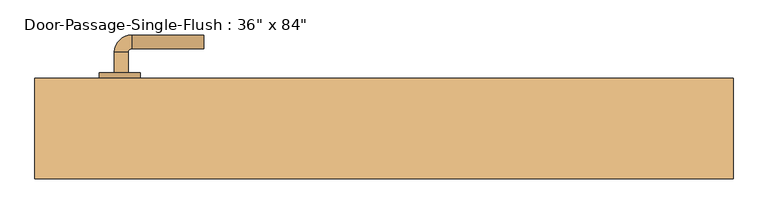
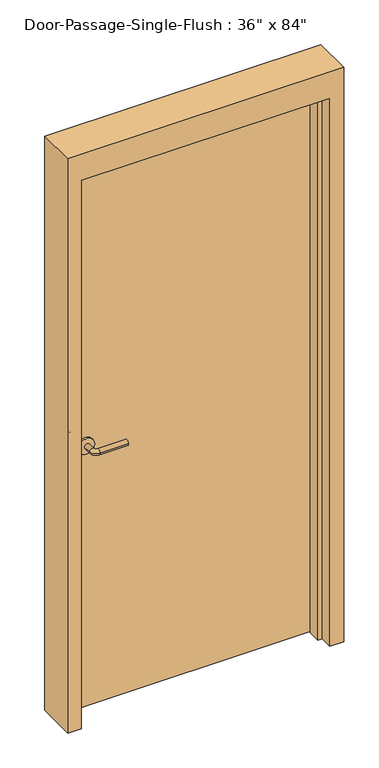
"""IFC4 building model written with IfcOpenShell, lengths in millimetres: door geometry."""

import ifcopenshell
import ifcopenshell.guid

model = None  # the IFC model being written
_history = None  # IfcOwnerHistory: only IFC2X3 demands one
_inside = {}  # id of a spatial element -> (the spatial element, [elements in it])
_under = {}  # id of a project, library or spatial element -> (it, [spatial elements below it])
_declared = {}  # id of a project -> (the project, [libraries it declares])
_typed = {}  # id of a type object -> (the type object, [elements of that type])
_made_of = {}  # id of a material, layer set ... -> (it, [elements and type objects made of it])


def new_model(schema):
    """Start an empty IFC model of exactly this schema.

    Asked for "IFC4X3", IfcOpenShell would pick the latest addendum, in which some entities
    have other attributes; the version numbers below select the first issue.
    IFC2X3 requires an IfcOwnerHistory on every rooted entity: one is made here for all.
    """
    global model, _history
    if schema == "IFC4X3":
        model = ifcopenshell.file(schema_version=(4, 3, 0, 0))
    else:
        model = ifcopenshell.file(schema=schema)
    _inside.clear()
    _under.clear()
    _declared.clear()
    _typed.clear()
    _made_of.clear()
    _history = None
    if model.schema == "IFC2X3":
        org = make("IfcOrganization", Name="unknown")
        user = make(
            "IfcPersonAndOrganization",
            ThePerson=make("IfcPerson", FamilyName="unknown"),
            TheOrganization=org,
        )
        app = make(
            "IfcApplication",
            ApplicationDeveloper=org,
            Version="unknown",
            ApplicationFullName="unknown",
            ApplicationIdentifier="unknown",
        )
        _history = make(
            "IfcOwnerHistory",
            OwningUser=user,
            OwningApplication=app,
            ChangeAction="ADDED",
            CreationDate=0,
        )
    return model


def make(cls, **values):
    """One entity of the class cls with the attributes given. An attribute that is None is left unset."""
    return model.create_entity(
        cls, **{name: value for name, value in values.items() if value is not None}
    )


def rooted(cls, **values):
    """An entity with a GlobalId (a new one), such as an element, a storey or a relation."""
    return make(cls, GlobalId=ifcopenshell.guid.new(), OwnerHistory=_history, **values)


def si_unit(unit_type, name, prefix=None):
    """IfcSIUnit, for example si_unit("LENGTHUNIT", "METRE", prefix="MILLI")."""
    return make("IfcSIUnit", UnitType=unit_type, Prefix=prefix, Name=name)


def assignment(units):
    """IfcUnitAssignment: the units of a project."""
    return None if units is None else make("IfcUnitAssignment", Units=units)


def point(xyz):
    """IfcCartesianPoint."""
    return None if xyz is None else make("IfcCartesianPoint", Coordinates=xyz)


def direction(xyz):
    """IfcDirection."""
    return None if xyz is None else make("IfcDirection", DirectionRatios=xyz)


def frame(location, z_axis=None, x_axis=None):
    """IfcAxis2Placement3D, a coordinate frame: its origin and axes. An axis left out is left unset."""
    return make(
        "IfcAxis2Placement3D",
        Location=point(location),
        Axis=direction(z_axis),
        RefDirection=direction(x_axis),
    )


def frame_2d(location, x_axis=None):
    """IfcAxis2Placement2D, a coordinate frame in the plane: its origin and x axis."""
    return make(
        "IfcAxis2Placement2D", Location=point(location), RefDirection=direction(x_axis)
    )


def origin():
    """The frame at (0, 0, 0) with its axes left unset."""
    return frame((0.0, 0.0, 0.0))


def origin_with_axes():
    """The frame at (0, 0, 0) with the z axis (0, 0, 1) and the x axis (1, 0, 0) written out."""
    return frame((0.0, 0.0, 0.0), z_axis=(0.0, 0.0, 1.0), x_axis=(1.0, 0.0, 0.0))


def place(relative_to, where):
    """IfcLocalPlacement: puts the frame where relative to a parent placement (None: the world)."""
    return make(
        "IfcLocalPlacement", PlacementRelTo=relative_to, RelativePlacement=where
    )


def context(
    kind, dimensions, precision=None, world=None, true_north=None, identifier=None
):
    """IfcGeometricRepresentationContext, for example the 3D "Model" context."""
    return make(
        "IfcGeometricRepresentationContext",
        ContextIdentifier=identifier,
        ContextType=kind,
        CoordinateSpaceDimension=dimensions,
        Precision=precision,
        WorldCoordinateSystem=world,
        TrueNorth=true_north,
    )


def project(units=None, contexts=None):
    """IfcProject with its units and contexts."""
    return rooted(
        "IfcProject",
        Name="project",
        RepresentationContexts=contexts,
        UnitsInContext=assignment(units),
    )


def spatial(cls, under=None, at=None, **own):
    """A site, building, storey or space (cls), placed at a placement, below another one or the project."""
    s = rooted(cls, ObjectPlacement=at, **own)
    if under is not None:
        _under.setdefault(under.id(), (under, []))[1].append(s)
    return s


def polyline(points):
    """IfcPolyline through the points."""
    return make("IfcPolyline", Points=[point(p) for p in points])


def circle_curve(where, radius):
    """IfcCircle in the frame where."""
    return make("IfcCircle", Position=where, Radius=radius)


def ellipse_curve(where, semi_axis1, semi_axis2):
    """IfcEllipse in the frame where."""
    return make(
        "IfcEllipse", Position=where, SemiAxis1=semi_axis1, SemiAxis2=semi_axis2
    )


def trimmed(basis, trim1, trim2, sense, master):
    """IfcTrimmedCurve: the piece of a basis curve between two trims."""
    return make(
        "IfcTrimmedCurve",
        BasisCurve=basis,
        Trim1=trim1,
        Trim2=trim2,
        SenseAgreement=sense,
        MasterRepresentation=master,
    )


def segment(curve, same_sense, transition):
    """IfcCompositeCurveSegment."""
    return make(
        "IfcCompositeCurveSegment",
        Transition=transition,
        SameSense=same_sense,
        ParentCurve=curve,
    )


def composite_curve(segments, self_intersect=None):
    """IfcCompositeCurve: segments joined end to end."""
    return make("IfcCompositeCurve", Segments=segments, SelfIntersect=self_intersect)


def outline(outer, holes=None, kind="AREA"):
    """IfcArbitraryClosedProfileDef: a profile drawn as a closed curve; with holes, ...WithVoids."""
    if holes is None:
        return make("IfcArbitraryClosedProfileDef", ProfileType=kind, OuterCurve=outer)
    return make(
        "IfcArbitraryProfileDefWithVoids",
        ProfileType=kind,
        OuterCurve=outer,
        InnerCurves=holes,
    )


def extrude(swept, where, along, depth):
    """IfcExtrudedAreaSolid: the profile swept, set in the frame where, extruded along a direction by depth."""
    return make(
        "IfcExtrudedAreaSolid",
        SweptArea=swept,
        Position=where,
        ExtrudedDirection=direction(along),
        Depth=depth,
    )


def faces_of(points, faces, orient=None, outer=None):
    """IfcFace entities. A face is a list of loops; a loop is a list of indices into points, from 0.

    orient and outer hold one flag for each loop. By default every Orientation is true, the
    first loop of a face is its IfcFaceOuterBound and the others are IfcFaceBound.
    """
    made = []
    for i, loops in enumerate(faces):
        bounds = []
        for j, loop in enumerate(loops):
            is_outer = j == 0 if outer is None else outer[i][j]
            bounds.append(
                make(
                    "IfcFaceOuterBound" if is_outer else "IfcFaceBound",
                    Bound=make("IfcPolyLoop", Polygon=[points[k] for k in loop]),
                    Orientation=True if orient is None else orient[i][j],
                )
            )
        made.append(make("IfcFace", Bounds=bounds))
    return made


def faceted_brep(points, faces, orient=None, outer=None, voids=None):
    """IfcFacetedBrep: a solid bounded by flat faces; with voids (closed shells), ...WithVoids."""
    shared = [point(p) for p in points]
    hull = make("IfcClosedShell", CfsFaces=faces_of(shared, faces, orient, outer))
    if voids is None:
        return make("IfcFacetedBrep", Outer=hull)
    return make(
        "IfcFacetedBrepWithVoids",
        Outer=hull,
        Voids=[
            make(cls, CfsFaces=faces_of(shared, fs, o, b)) for cls, fs, o, b in voids
        ],
    )


def shape(context_of_items, identifier, shape_type, items):
    """IfcShapeRepresentation: the items that make up one representation, for example the "Body"."""
    return make(
        "IfcShapeRepresentation",
        ContextOfItems=context_of_items,
        RepresentationIdentifier=identifier,
        RepresentationType=shape_type,
        Items=items,
    )


def source(mapping_origin, context_of_items, identifier, shape_type, items):
    """IfcRepresentationMap: a shape defined once, which mapped items show again and again."""
    return make(
        "IfcRepresentationMap",
        MappingOrigin=mapping_origin,
        MappedRepresentation=shape(context_of_items, identifier, shape_type, items),
    )


def transform(
    local_origin,
    x_axis=None,
    y_axis=None,
    z_axis=None,
    scale=None,
    scale2=None,
    scale3=None,
    uniform=True,
):
    """IfcCartesianTransformationOperator3D, or its non-uniform kind. x_axis, y_axis, z_axis: its Axis1, 2, 3."""
    if uniform:
        return make(
            "IfcCartesianTransformationOperator3D",
            Axis1=direction(x_axis),
            Axis2=direction(y_axis),
            LocalOrigin=point(local_origin),
            Scale=scale,
            Axis3=direction(z_axis),
        )
    return make(
        "IfcCartesianTransformationOperator3DnonUniform",
        Axis1=direction(x_axis),
        Axis2=direction(y_axis),
        LocalOrigin=point(local_origin),
        Scale=scale,
        Axis3=direction(z_axis),
        Scale2=scale2,
        Scale3=scale3,
    )


def mapped(mapping_source, mapping_target):
    """IfcMappedItem: shows the shape of a source again, moved by a transform."""
    return make(
        "IfcMappedItem", MappingSource=mapping_source, MappingTarget=mapping_target
    )


def made_of(thing, what):
    """Note that an element or type object is made of a material, layer set ...; save() writes the relation."""
    if what is not None:
        _made_of.setdefault(what.id(), (what, []))[1].append(thing)
    return thing


def element(
    cls,
    number,
    at=None,
    inside=None,
    cuts=None,
    type_object=None,
    material=None,
    context=None,
    identifier="Body",
    shape_type=None,
    held_by="IfcProductDefinitionShape",
    body=None,
    shapes=None,
    **own,
):
    """One element of the class cls, such as IfcWall. Its Tag is "e" and its number.

    at: its placement. inside: the storey or other place that contains it. cuts: it is an
    opening in that element (IfcRelVoidsElement). A single representation is given by context,
    identifier, shape_type and body (its items); several are given by shapes. held_by: the class
    of the entity that holds the representations. save() writes the other relations.
    """
    e = rooted(cls, Tag="e%d" % number, ObjectPlacement=at, **own)
    if body is not None:
        shapes = [shape(context, identifier, shape_type, body)]
    if shapes is not None:
        e.Representation = make(held_by, Representations=shapes)
    if inside is not None:
        _inside.setdefault(inside.id(), (inside, []))[1].append(e)
    if cuts is not None:
        rooted(
            "IfcRelVoidsElement", RelatingBuildingElement=cuts, RelatedOpeningElement=e
        )
    if type_object is not None:
        _typed.setdefault(type_object.id(), (type_object, []))[1].append(e)
    return made_of(e, material)


def aggregate(whole, parts):
    """IfcRelAggregates: a whole, such as a stair, and the parts it consists of."""
    return rooted("IfcRelAggregates", RelatingObject=whole, RelatedObjects=parts)


def save(model, path):
    """Write the relations noted so far, then the file.

    IfcRelAggregates (storeys below a building ...), IfcRelContainedInSpatialStructure (elements
    in a storey), IfcRelDefinesByType, IfcRelAssociatesMaterial and IfcRelDeclares: one each for
    every whole, place, type object, material and project.
    """
    for whole, parts in _under.values():
        aggregate(whole, parts)
    for where, things in _inside.values():
        rooted(
            "IfcRelContainedInSpatialStructure",
            RelatedElements=things,
            RelatingStructure=where,
        )
    for kind, things in _typed.values():
        rooted("IfcRelDefinesByType", RelatedObjects=things, RelatingType=kind)
    for what, things in _made_of.values():
        rooted("IfcRelAssociatesMaterial", RelatedObjects=things, RelatingMaterial=what)
    for by, libraries in _declared.values():
        rooted("IfcRelDeclares", RelatingContext=by, RelatedDefinitions=libraries)
    model.write(path)


def plane_surface(at):
    """IfcPlane: the flat surface through the origin of the frame at, square to its z axis."""
    return make("IfcPlane", Position=at)


def cylinder_surface(at, radius):
    """IfcCylindricalSurface: all points at the distance radius from the z axis of the frame at."""
    return make("IfcCylindricalSurface", Position=at, Radius=radius)


def revolved_surface(curve, axis_point, axis_direction):
    """IfcSurfaceOfRevolution: the curve turned about the line through axis_point along axis_direction."""
    return make(
        "IfcSurfaceOfRevolution",
        SweptCurve=make("IfcArbitraryOpenProfileDef", ProfileType="CURVE", Curve=curve),
        AxisPosition=make("IfcAxis1Placement", Location=point(axis_point), Axis=direction(axis_direction)),
    )


def advanced_brep(points, edges, surfaces, faces):
    """IfcAdvancedBrep: a solid bounded by faces that lie on surfaces and meet in shared edges.

    An edge is (start, end): straight between two places in points (the first is 0);
    or (start, end, curve); or (start, end, curve, False) where it runs against its curve.
    A face is (place in surfaces, loops), or (place, loops, False) where it looks against
    its surface's normal. A loop lists edges by number (the first is 1), with a minus sign
    where the edge is run from its end to its start. The first loop is the outer one.
    """
    corners = [point(p) for p in points]
    vertices = [make("IfcVertexPoint", VertexGeometry=c) for c in corners]
    made = []
    for start, end, *more in edges:
        made.append(
            make(
                "IfcEdgeCurve",
                EdgeStart=vertices[start],
                EdgeEnd=vertices[end],
                EdgeGeometry=more[0] if more else make("IfcPolyline", Points=[corners[start], corners[end]]),
                SameSense=more[1] if len(more) > 1 else True,
            )
        )
    hull = []
    for where, loops, *sense in faces:
        bounds = []
        for j, loop in enumerate(loops):
            ring = [make("IfcOrientedEdge", EdgeElement=made[abs(k) - 1], Orientation=k > 0) for k in loop]
            bounds.append(
                make(
                    "IfcFaceOuterBound" if j == 0 else "IfcFaceBound",
                    Bound=make("IfcEdgeLoop", EdgeList=ring),
                    Orientation=True,
                )
            )
        hull.append(make("IfcAdvancedFace", Bounds=bounds, FaceSurface=surfaces[where], SameSense=sense[0] if sense else True))
    return make("IfcAdvancedBrep", Outer=make("IfcClosedShell", CfsFaces=hull))


def door_a255baf1(model_context):
    return source(origin(), model_context, "Body", "SolidModel", [
        advanced_brep(
        [(-392.190625, -1.65, 1016.0), (-372.190625, -1.65, 1016.0), (-372.190625, -31.65, 1016.0), (-392.190625, -31.65, 1016.0), (-367.190625, -36.65, 1016.0), (-367.190625, -56.65, 1016.0), (-262.190625, -56.65, 1016.0), (-262.190625, -36.65, 1016.0)],
        [
            (0, 1, circle_curve(frame((-382.190625, -1.65, 1016.0), z_axis=(0.0, 1.0, 0.0), x_axis=(1.0, 0.0, 0.0)), 10.0)),
            (1, 0, circle_curve(frame((-382.190625, -1.65, 1016.0), z_axis=(0.0, 1.0, 0.0), x_axis=(1.0, 0.0, 0.0)), 10.0)),
            (1, 2),
            (2, 3, circle_curve(frame((-382.190625, -31.65, 1016.0), z_axis=(0.0, 1.0, 0.0), x_axis=(1.0, 0.0, 0.0)), 10.0)),
            (3, 0),
            (3, 2, circle_curve(frame((-382.190625, -31.65, 1016.0), z_axis=(0.0, 1.0, 0.0), x_axis=(1.0, 0.0, 0.0)), 10.0)),
            (4, 5, circle_curve(frame((-367.190625, -46.65, 1016.0), z_axis=(-1.0, 0.0, 0.0), x_axis=(0.0, 1.0, 0.0)), 10.0)),
            (5, 3, circle_curve(frame((-367.190625, -31.65, 1016.0), z_axis=(0.0, 0.0, -1.0), x_axis=(-1.0, 0.0, 0.0)), 25.0)),
            (2, 4, circle_curve(frame((-367.190625, -31.65, 1016.0), z_axis=(0.0, 0.0, 1.0), x_axis=(-1.0, 0.0, 0.0)), 5.0)),
            (5, 4, circle_curve(frame((-367.190625, -46.65, 1016.0), z_axis=(-1.0, 0.0, 0.0), x_axis=(0.0, 1.0, 0.0)), 10.0)),
            (6, 7, circle_curve(frame((-262.190625, -46.65, 1016.0), z_axis=(1.0, 0.0, 0.0), x_axis=(0.0, 1.0, 0.0)), 10.0)),
            (7, 6, circle_curve(frame((-262.190625, -46.65, 1016.0), z_axis=(1.0, 0.0, 0.0), x_axis=(0.0, 1.0, 0.0)), 10.0)),
            (4, 7),
            (6, 5),
        ],
        [
            plane_surface(frame((-382.190625, -1.65, 1016.0), z_axis=(0.0, 1.0, 0.0), x_axis=(0.0, 0.0, 1.0))),
            cylinder_surface(frame((-382.190625, -1.65, 1016.0), z_axis=(0.0, 1.0, 0.0), x_axis=(1.0, 0.0, 0.0)), 10.0),
            revolved_surface(trimmed(ellipse_curve(frame((-382.190625, -31.65, 1016.0), z_axis=(0.0, -1.0, 0.0), x_axis=(1.0, 0.0, 0.0)), 10.0, 10.0), [point((-392.190625, -31.65, 1016.0))], [point((-372.190625, -31.65, 1016.0))], True, "CARTESIAN"), (-367.190625, -31.65, 1016.0), (0.0, 0.0, -1.0)),
            revolved_surface(trimmed(ellipse_curve(frame((-382.190625, -31.65, 1016.0), z_axis=(0.0, -1.0, 0.0), x_axis=(1.0, 0.0, 0.0)), 10.0, 10.0), [point((-372.190625, -31.65, 1016.0))], [point((-392.190625, -31.65, 1016.0))], True, "CARTESIAN"), (-367.190625, -31.65, 1016.0), (0.0, 0.0, -1.0)),
            plane_surface(frame((-262.190625, -46.65, 1016.0), z_axis=(1.0, 0.0, 0.0), x_axis=(0.0, 0.0, 1.0))),
            cylinder_surface(frame((-367.190625, -46.65, 1016.0), z_axis=(-1.0, 0.0, 0.0), x_axis=(0.0, 1.0, 0.0)), 10.0),
        ],
        [
            (0, [[1, 2]]),
            (1, [[3, 4, 5, -2]]),
            (1, [[-5, 6, -3, -1]]),
            (2, [[7, 8, -4, 9]]),
            (3, [[10, -9, -6, -8]]),
            (4, [[11, 12]]),
            (5, [[13, -11, 14, -7]]),
            (5, [[-14, -12, -13, -10]]),
        ],
    ),
        extrude(outline(composite_curve([segment(trimmed(circle_curve(frame_2d((1016.0, -384.690625)), 30.0), [point((1016.0, -414.690625))], [point((1016.0, -354.690625))], False, "CARTESIAN"), True, "CONTINUOUS"), segment(trimmed(circle_curve(frame_2d((1016.0, -384.690625)), 30.0), [point((1016.0, -354.690625))], [point((1016.0, -414.690625))], False, "CARTESIAN"), True, "CONTINUOUS")], self_intersect=False)), frame((0.0, -1.65, 0.0), z_axis=(0.0, 1.0, 0.0), x_axis=(0.0, 0.0, 1.0)), (0.0, 0.0, 1.0), 8.0),
        advanced_brep(
        [(-392.190625, 58.8, 1016.0), (-372.190625, 58.8, 1016.0), (-392.190625, 88.8, 1016.0), (-372.190625, 88.8, 1016.0), (-367.190625, 93.8, 1016.0), (-367.190625, 113.8, 1016.0), (-262.190625, 113.8, 1016.0), (-262.190625, 93.8, 1016.0)],
        [
            (0, 1, circle_curve(frame((-382.190625, 58.8, 1016.0), z_axis=(0.0, -1.0, 0.0), x_axis=(1.0, 0.0, 0.0)), 10.0)),
            (1, 0, circle_curve(frame((-382.190625, 58.8, 1016.0), z_axis=(0.0, -1.0, 0.0), x_axis=(1.0, 0.0, 0.0)), 10.0)),
            (0, 2),
            (2, 3, circle_curve(frame((-382.190625, 88.8, 1016.0), z_axis=(0.0, -1.0, 0.0), x_axis=(1.0, 0.0, 0.0)), 10.0)),
            (3, 1),
            (3, 2, circle_curve(frame((-382.190625, 88.8, 1016.0), z_axis=(0.0, -1.0, 0.0), x_axis=(1.0, 0.0, 0.0)), 10.0)),
            (4, 3, circle_curve(frame((-367.190625, 88.8, 1016.0), z_axis=(0.0, 0.0, 1.0), x_axis=(-1.0, 0.0, 0.0)), 5.0)),
            (2, 5, circle_curve(frame((-367.190625, 88.8, 1016.0), z_axis=(0.0, 0.0, -1.0), x_axis=(-1.0, 0.0, 0.0)), 25.0)),
            (5, 4, circle_curve(frame((-367.190625, 103.8, 1016.0), z_axis=(-1.0, 0.0, 0.0), x_axis=(0.0, -1.0, 0.0)), 10.0)),
            (4, 5, circle_curve(frame((-367.190625, 103.8, 1016.0), z_axis=(-1.0, 0.0, 0.0), x_axis=(0.0, -1.0, 0.0)), 10.0)),
            (6, 7, circle_curve(frame((-262.190625, 103.8, 1016.0), z_axis=(1.0, 0.0, 0.0), x_axis=(0.0, -1.0, 0.0)), 10.0)),
            (7, 6, circle_curve(frame((-262.190625, 103.8, 1016.0), z_axis=(1.0, 0.0, 0.0), x_axis=(0.0, -1.0, 0.0)), 10.0)),
            (5, 6),
            (7, 4),
        ],
        [
            plane_surface(frame((-382.190625, 58.8, 1016.0), z_axis=(0.0, -1.0, 0.0), x_axis=(0.0, 0.0, 1.0))),
            cylinder_surface(frame((-382.190625, 58.8, 1016.0), z_axis=(0.0, -1.0, 0.0), x_axis=(1.0, 0.0, 0.0)), 10.0),
            revolved_surface(trimmed(ellipse_curve(frame((-382.190625, 88.8, 1016.0), z_axis=(0.0, -1.0, 0.0), x_axis=(1.0, 0.0, 0.0)), 10.0, 10.0), [point((-392.190625, 88.8, 1016.0))], [point((-372.190625, 88.8, 1016.0))], True, "CARTESIAN"), (-367.190625, 88.8, 1016.0), (0.0, 0.0, -1.0)),
            revolved_surface(trimmed(ellipse_curve(frame((-382.190625, 88.8, 1016.0), z_axis=(0.0, -1.0, 0.0), x_axis=(1.0, 0.0, 0.0)), 10.0, 10.0), [point((-372.190625, 88.8, 1016.0))], [point((-392.190625, 88.8, 1016.0))], True, "CARTESIAN"), (-367.190625, 88.8, 1016.0), (0.0, 0.0, -1.0)),
            plane_surface(frame((-262.190625, 103.8, 1016.0), z_axis=(1.0, 0.0, 0.0), x_axis=(0.0, 0.0, 1.0))),
            cylinder_surface(frame((-367.190625, 103.8, 1016.0), z_axis=(-1.0, 0.0, 0.0), x_axis=(0.0, -1.0, 0.0)), 10.0),
        ],
        [
            (0, [[1, 2]]),
            (1, [[-1, 3, 4, 5]]),
            (1, [[-2, -5, 6, -3]]),
            (2, [[7, -4, 8, 9]]),
            (3, [[-8, -6, -7, 10]]),
            (4, [[11, 12]]),
            (5, [[-9, 13, -12, 14]]),
            (5, [[-10, -14, -11, -13]]),
        ],
    ),
        extrude(outline(composite_curve([segment(trimmed(circle_curve(frame_2d((1016.0, -384.690625)), 30.0), [point((1016.0, -414.690625))], [point((1016.0, -354.690625))], False, "CARTESIAN"), True, "CONTINUOUS"), segment(trimmed(circle_curve(frame_2d((1016.0, -384.690625)), 30.0), [point((1016.0, -354.690625))], [point((1016.0, -414.690625))], False, "CARTESIAN"), True, "CONTINUOUS")], self_intersect=False)), frame((0.0, 50.8, 0.0), z_axis=(0.0, 1.0, 0.0), x_axis=(0.0, 0.0, 1.0)), (0.0, 0.0, 1.0), 8.0),
        faceted_brep([(457.2, 1.5875, 0.0), (457.2, 50.8, 0.0), (508.0, 50.8, 0.0), (508.0, -95.25, 0.0), (457.2, -95.25, 0.0), (457.2, -46.0375, 0.0), (441.325, -46.0375, 0.0), (441.325, 1.5875, 0.0), (457.2, 1.5875, 2133.6), (457.2, 50.8, 2133.6), (-457.2, 50.8, 2133.6), (-457.2, 50.8, 0.0), (-508.0, 50.8, 0.0), (-508.0, 50.8, 2235.2), (508.0, 50.8, 2235.2), (508.0, -95.25, 2235.2), (-508.0, -95.25, 2235.2), (-508.0, -95.25, 0.0), (-457.2, -95.25, 0.0), (-457.2, -95.25, 2133.6), (457.2, -95.25, 2133.6), (457.2, -46.0375, 2133.6), (-457.2, -46.0375, 2133.6), (-457.2, -46.0375, 0.0), (-441.325, -46.0375, 0.0), (-441.325, -46.0375, 2117.725), (441.325, -46.0375, 2117.725), (441.325, 1.5875, 2117.725), (-441.325, 1.5875, 2117.725), (-441.325, 1.5875, 0.0), (-457.2, 1.5875, 0.0), (-457.2, 1.5875, 2133.6)], [[[0, 1, 2, 3, 4, 5, 6, 7]], [[1, 0, 8, 9]], [[2, 1, 9, 10, 11, 12, 13, 14]], [[3, 2, 14, 15]], [[4, 3, 15, 16, 17, 18, 19, 20]], [[5, 4, 20, 21]], [[6, 5, 21, 22, 23, 24, 25, 26]], [[7, 6, 26, 27]], [[0, 7, 27, 28, 29, 30, 31, 8]], [[9, 8, 31, 10]], [[20, 19, 22, 21]], [[26, 25, 28, 27]], [[12, 11, 30, 29, 24, 23, 18, 17]], [[11, 10, 31, 30]], [[13, 12, 17, 16]], [[19, 18, 23, 22]], [[25, 24, 29, 28]], [[15, 14, 13, 16]]]),
        extrude(outline(polyline([(457.2, 6.35), (-457.2, 6.35), (-457.2, 50.8), (457.2, 50.8), (457.2, 6.35)])), origin_with_axes(), (0.0, 0.0, 1.0), 2133.6),
    ])


if __name__ == "__main__":
    model = new_model("IFC4")
    model_context = context("Model", 3, world=origin())
    ifc_project = project(units=[si_unit("LENGTHUNIT", "METRE", prefix="MILLI")], contexts=[model_context])
    site = spatial("IfcSite", under=ifc_project)
    building = spatial("IfcBuilding", under=site)
    placement = place(None, origin())
    door_shape = door_a255baf1(model_context)
    element("IfcDoor", 1, ObjectType="Door-Passage-Single-Flush : 36\" x 84\"", at=placement, inside=building, context=model_context, shape_type="MappedRepresentation", body=[
        mapped(door_shape, transform((0.0, 0.0, 0.0), x_axis=(1.0, 0.0, 0.0), y_axis=(0.0, 1.0, 0.0), z_axis=(0.0, 0.0, 1.0))),
    ])
    save(model, "model.ifc")

# Revit data of these elements
# Type "Door-Passage-Single-Flush : 36\" x 84\""
#   Type Mark = "35"
#   Assembly Code = "B2030200"
#   Analytic Construction = "Wooden"
#   Thickness = 0' - 1 3/4"
#   Thermal Resistance (R) = 2.5876 (h·ft²·°F)/BTU
#   Swing Angle [instance default] = 90.00°
#   Strike Height = 3' - 4"
#   Rough Width [instance default] = 3' - 4"
#   Rough Height [instance default] = 7' - 4"
#   MF Opening Height [instance default] = 0' - 4"
#   MF Opening Width [instance default] = 0' - 4"
#   Inset Calculate [instance default] = 0' - 4"
#   Masonry Inset [instance default] = 0' - 1"
#   Height = 7' - 0"
#   Width = 3' - 0"
#   Heat Transfer Coefficient (U) = 0.3865 BTU/(h·ft²·°F)
#   Masonry Frame Depth = 0' - 5 3/4"
#   Masonry Frame [instance default] = yes
#   Function = 1
#   Dry Wall Frame [instance default] = no
#   Panel Material = Wood - Birch
#   Frame Material = Metal - Paint Finish - Grey
#   Door Handle Material = Aluminum
#   Visual Light Transmittance = 0
#   Solar Heat Gain Coefficient = 0
#   Wall Closure = (empty or 0)
# Element 1 (IfcDoor, "Door-Passage-Single-Flush : 36\" x 84\"")
#   Materials on its faces: "Aluminum", "Metal - Paint Finish - Grey", "Wood - Birch"
# Materials
#   "Wood - Birch": class "Wood", colour RGB 166 116 52, transparency 0, Cost = 0
#   "Metal - Paint Finish - Grey": class "Paint", colour RGB 104 104 104, transparency 0, Cost = 0
#   "Aluminum": class "Metal", colour RGB 247 247 247, transparency 0, Description = "Aluminum 6061", Cost = 0
